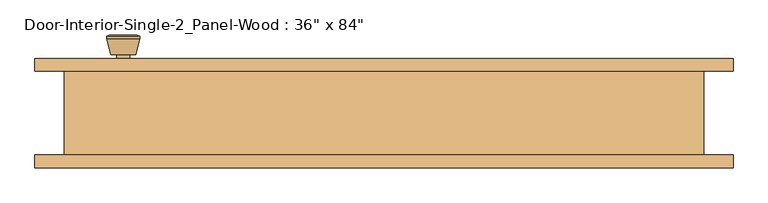
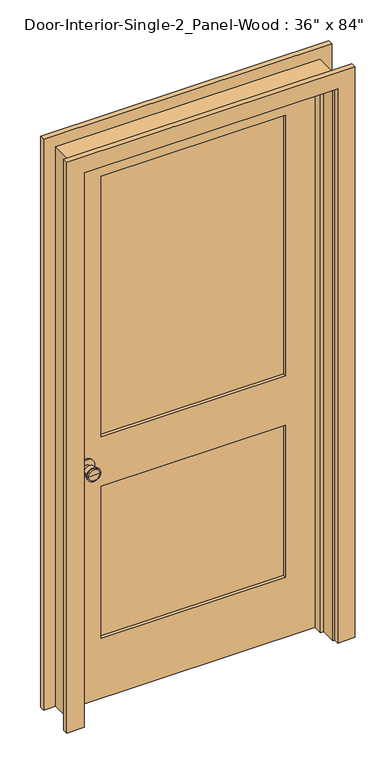
"""IFC4 building model written with IfcOpenShell, lengths in millimetres: door geometry."""

from ifc_helpers import new_model, si_unit, point, frame, frame_2d, origin, place, context, project, spatial, polyline, circle_curve, trimmed, segment, composite_curve, outline, extrude, faceted_brep, source, transform, mapped, element, save
from ifc_brep_helpers import plane_surface, cylinder_surface, revolved_surface, advanced_brep


def door_9f0e9c7d(model_context):
    return source(origin(), model_context, "Body", "SolidModel", [
        advanced_brep(
        [(-393.7, 19.4, 914.4), (-383.7, 19.4, 914.4), (-403.7, 19.4, 914.4), (-373.2241324, -29.6, 914.4), (-393.7, -29.6, 914.4), (-414.1758676, -29.6, 914.4), (-368.7, -27.7721319, 914.4), (-418.7, -27.7721319, 914.4), (-368.7, -24.3084537, 914.4), (-418.7, -24.3084537, 914.4), (-375.063764, 0.4, 914.4), (-412.336236, 0.4, 914.4), (-383.7, 0.4, 914.4), (-403.7, 0.4, 914.4)],
        [
            (0, 1),
            (1, 2, circle_curve(frame((-393.7, 19.4, 914.4), z_axis=(0.0, 1.0, 0.0), x_axis=(-1.0, 0.0, 0.0)), 10.0)),
            (2, 0),
            (2, 1, circle_curve(frame((-393.7, 19.4, 914.4), z_axis=(0.0, 1.0, 0.0), x_axis=(-1.0, 0.0, 0.0)), 10.0)),
            (3, 4),
            (4, 5),
            (5, 3, circle_curve(frame((-393.7, -29.6, 914.4), z_axis=(0.0, -1.0, 0.0), x_axis=(-1.0, 0.0, 0.0)), 20.4758676)),
            (3, 5, circle_curve(frame((-393.7, -29.6, 914.4), z_axis=(0.0, -1.0, 0.0), x_axis=(-1.0, 0.0, 0.0)), 20.4758676)),
            (6, 3),
            (5, 7),
            (7, 6, circle_curve(frame((-393.7, -27.7721319, 914.4), z_axis=(0.0, -1.0, 0.0), x_axis=(-1.0, 0.0, 0.0)), 25.0)),
            (6, 7, circle_curve(frame((-393.7, -27.7721319, 914.4), z_axis=(0.0, -1.0, 0.0), x_axis=(-1.0, 0.0, 0.0)), 25.0)),
            (8, 6),
            (7, 9),
            (9, 8, circle_curve(frame((-393.7, -24.3084537, 914.4), z_axis=(0.0, -1.0, 0.0), x_axis=(-1.0, 0.0, 0.0)), 25.0)),
            (8, 9, circle_curve(frame((-393.7, -24.3084537, 914.4), z_axis=(0.0, -1.0, 0.0), x_axis=(-1.0, 0.0, 0.0)), 25.0)),
            (10, 8),
            (9, 11),
            (11, 10, circle_curve(frame((-393.7, 0.4, 914.4), z_axis=(0.0, -1.0, 0.0), x_axis=(-1.0, 0.0, 0.0)), 18.636236)),
            (10, 11, circle_curve(frame((-393.7, 0.4, 914.4), z_axis=(0.0, -1.0, 0.0), x_axis=(-1.0, 0.0, 0.0)), 18.636236)),
            (12, 10),
            (11, 13),
            (13, 12, circle_curve(frame((-393.7, 0.4, 914.4), z_axis=(0.0, -1.0, 0.0), x_axis=(-1.0, 0.0, 0.0)), 10.0)),
            (12, 13, circle_curve(frame((-393.7, 0.4, 914.4), z_axis=(0.0, -1.0, 0.0), x_axis=(-1.0, 0.0, 0.0)), 10.0)),
            (1, 12),
            (13, 2),
        ],
        [
            plane_surface(frame((-393.7, 19.4, 914.4), z_axis=(0.0, 1.0, 0.0), x_axis=(-1.0, 0.0, 0.0))),
            plane_surface(frame((-393.7, -29.6, 914.4), z_axis=(0.0, -1.0, 0.0), x_axis=(-1.0, 0.0, 0.0))),
            revolved_surface(polyline([(-414.1758676, -29.6, 914.4), (-418.7, -27.7721319, 914.4)]), (-393.7, 19.4, 914.4), (0.0, 1.0, 0.0)),
            cylinder_surface(frame((-393.7, 19.4, 914.4), z_axis=(0.0, 1.0, 0.0), x_axis=(-1.0, 0.0, 0.0)), 25.0),
            revolved_surface(polyline([(-418.7, -24.3084537, 914.4), (-412.336236, 0.4, 914.4)]), (-393.7, 19.4, 914.4), (0.0, 1.0, 0.0)),
            plane_surface(frame((-393.7, 0.4, 914.4), z_axis=(0.0, 1.0, 0.0), x_axis=(-1.0, 0.0, 0.0))),
            cylinder_surface(frame((-393.7, 19.4, 914.4), z_axis=(0.0, 1.0, 0.0), x_axis=(-1.0, 0.0, 0.0)), 10.0),
        ],
        [
            (0, [[1, 2, 3]]),
            (0, [[-3, 4, -1]]),
            (1, [[5, 6, 7]]),
            (1, [[-6, -5, 8]]),
            (2, [[9, -7, 10, 11]]),
            (2, [[-10, -8, -9, 12]]),
            (3, [[13, -11, 14, 15]]),
            (3, [[-14, -12, -13, 16]]),
            (4, [[17, -15, 18, 19]]),
            (4, [[-18, -16, -17, 20]]),
            (5, [[21, -19, 22, 23]]),
            (5, [[-22, -20, -21, 24]]),
            (6, [[25, -23, 26, -2]]),
            (6, [[-26, -24, -25, -4]]),
        ],
    ),
        extrude(outline(composite_curve([segment(trimmed(circle_curve(frame_2d((914.4, -393.7)), 30.0), [point((914.4, -423.7))], [point((914.4, -363.7))], False, "CARTESIAN"), True, "CONTINUOUS"), segment(trimmed(circle_curve(frame_2d((914.4, -393.7)), 30.0), [point((914.4, -363.7))], [point((914.4, -423.7))], False, "CARTESIAN"), True, "CONTINUOUS")], self_intersect=False)), frame((0.0, 19.4, 0.0), z_axis=(0.0, 1.0, 0.0), x_axis=(0.0, 0.0, 1.0)), (0.0, 0.0, 1.0), 6.0),
        advanced_brep(
        [(-393.7, 66.325, 914.4), (-403.7, 66.325, 914.4), (-383.7, 66.325, 914.4), (-373.2241324, 115.325, 914.4), (-414.1758676, 115.325, 914.4), (-393.7, 115.325, 914.4), (-368.7, 113.4971319, 914.4), (-418.7, 113.4971319, 914.4), (-368.7, 110.0334537, 914.4), (-418.7, 110.0334537, 914.4), (-375.063764, 85.325, 914.4), (-412.336236, 85.325, 914.4), (-383.7, 85.325, 914.4), (-403.7, 85.325, 914.4)],
        [
            (0, 1),
            (1, 2, circle_curve(frame((-393.7, 66.325, 914.4), z_axis=(0.0, -1.0, 0.0), x_axis=(-1.0, 0.0, 0.0)), 10.0)),
            (2, 0),
            (2, 1, circle_curve(frame((-393.7, 66.325, 914.4), z_axis=(0.0, -1.0, 0.0), x_axis=(-1.0, 0.0, 0.0)), 10.0)),
            (3, 4, circle_curve(frame((-393.7, 115.325, 914.4), z_axis=(0.0, 1.0, 0.0), x_axis=(-1.0, 0.0, 0.0)), 20.4758676)),
            (4, 5),
            (5, 3),
            (4, 3, circle_curve(frame((-393.7, 115.325, 914.4), z_axis=(0.0, 1.0, 0.0), x_axis=(-1.0, 0.0, 0.0)), 20.4758676)),
            (6, 7, circle_curve(frame((-393.7, 113.4971319, 914.4), z_axis=(0.0, 1.0, 0.0), x_axis=(-1.0, 0.0, 0.0)), 25.0)),
            (7, 4),
            (3, 6),
            (7, 6, circle_curve(frame((-393.7, 113.4971319, 914.4), z_axis=(0.0, 1.0, 0.0), x_axis=(-1.0, 0.0, 0.0)), 25.0)),
            (8, 9, circle_curve(frame((-393.7, 110.0334537, 914.4), z_axis=(0.0, 1.0, 0.0), x_axis=(-1.0, 0.0, 0.0)), 25.0)),
            (9, 7),
            (6, 8),
            (9, 8, circle_curve(frame((-393.7, 110.0334537, 914.4), z_axis=(0.0, 1.0, 0.0), x_axis=(-1.0, 0.0, 0.0)), 25.0)),
            (10, 11, circle_curve(frame((-393.7, 85.325, 914.4), z_axis=(0.0, 1.0, 0.0), x_axis=(-1.0, 0.0, 0.0)), 18.636236)),
            (11, 9),
            (8, 10),
            (11, 10, circle_curve(frame((-393.7, 85.325, 914.4), z_axis=(0.0, 1.0, 0.0), x_axis=(-1.0, 0.0, 0.0)), 18.636236)),
            (12, 13, circle_curve(frame((-393.7, 85.325, 914.4), z_axis=(0.0, 1.0, 0.0), x_axis=(-1.0, 0.0, 0.0)), 10.0)),
            (13, 11),
            (10, 12),
            (13, 12, circle_curve(frame((-393.7, 85.325, 914.4), z_axis=(0.0, 1.0, 0.0), x_axis=(-1.0, 0.0, 0.0)), 10.0)),
            (1, 13),
            (12, 2),
        ],
        [
            plane_surface(frame((-393.7, 66.325, 914.4), z_axis=(0.0, -1.0, 0.0), x_axis=(-1.0, 0.0, 0.0))),
            plane_surface(frame((-393.7, 115.325, 914.4), z_axis=(0.0, 1.0, 0.0), x_axis=(-1.0, 0.0, 0.0))),
            revolved_surface(polyline([(-414.1758676, 115.325, 914.4), (-418.7, 113.4971319, 914.4)]), (-393.7, 66.325, 914.4), (0.0, -1.0, 0.0)),
            cylinder_surface(frame((-393.7, 66.325, 914.4), z_axis=(0.0, -1.0, 0.0), x_axis=(-1.0, 0.0, 0.0)), 25.0),
            revolved_surface(polyline([(-418.7, 110.0334537, 914.4), (-412.336236, 85.325, 914.4)]), (-393.7, 66.325, 914.4), (0.0, -1.0, 0.0)),
            plane_surface(frame((-393.7, 85.325, 914.4), z_axis=(0.0, -1.0, 0.0), x_axis=(-1.0, 0.0, 0.0))),
            cylinder_surface(frame((-393.7, 66.325, 914.4), z_axis=(0.0, -1.0, 0.0), x_axis=(-1.0, 0.0, 0.0)), 10.0),
        ],
        [
            (0, [[1, 2, 3]]),
            (0, [[-3, 4, -1]]),
            (1, [[5, 6, 7]]),
            (1, [[8, -7, -6]]),
            (2, [[9, 10, -5, 11]]),
            (2, [[12, -11, -8, -10]]),
            (3, [[13, 14, -9, 15]]),
            (3, [[16, -15, -12, -14]]),
            (4, [[17, 18, -13, 19]]),
            (4, [[20, -19, -16, -18]]),
            (5, [[21, 22, -17, 23]]),
            (5, [[24, -23, -20, -22]]),
            (6, [[-2, 25, -21, 26]]),
            (6, [[-4, -26, -24, -25]]),
        ],
    ),
        extrude(outline(composite_curve([segment(trimmed(circle_curve(frame_2d((914.4, -393.7)), 30.0), [point((914.4, -423.7))], [point((914.4, -363.7))], False, "CARTESIAN"), True, "CONTINUOUS"), segment(trimmed(circle_curve(frame_2d((914.4, -393.7)), 30.0), [point((914.4, -363.7))], [point((914.4, -423.7))], False, "CARTESIAN"), True, "CONTINUOUS")], self_intersect=False)), frame((0.0, 60.325, 0.0), z_axis=(0.0, 1.0, 0.0), x_axis=(0.0, 0.0, 1.0)), (0.0, 0.0, 1.0), 6.0),
        extrude(outline(polyline([(336.55, 37.0416667), (-336.55, 37.0416667), (-336.55, 48.6833333), (336.55, 48.6833333), (336.55, 37.0416667)])), frame((0.0, 0.0, 1009.65), z_axis=(0.0, 0.0, 1.0), x_axis=(1.0, 0.0, 0.0)), (0.0, 0.0, 1.0), 1004.8875),
        extrude(outline(polyline([(336.55, 37.0416667), (-336.55, 37.0416667), (-336.55, 48.6833333), (336.55, 48.6833333), (336.55, 37.0416667)])), frame((0.0, 0.0, 231.775), z_axis=(0.0, 0.0, 1.0), x_axis=(1.0, 0.0, 0.0)), (0.0, 0.0, 1.0), 587.375),
        extrude(outline(polyline([(2133.6, -457.2), (0.0, -457.2), (0.0, 457.2), (2133.6, 457.2), (2133.6, -457.2)]), holes=[polyline([(2014.5375, -336.55), (2014.5375, 336.55), (1009.65, 336.55), (1009.65, -336.55), (2014.5375, -336.55)]), polyline([(819.15, -336.55), (819.15, 336.55), (231.775, 336.55), (231.775, -336.55), (819.15, -336.55)])]), frame((0.0, 25.4, 0.0), z_axis=(0.0, 1.0, 0.0), x_axis=(0.0, 0.0, 1.0)), (0.0, 0.0, 1.0), 34.925),
        faceted_brep([(482.6, 60.325, 0.0), (482.6, -66.675, 0.0), (457.2, -66.675, 0.0), (457.2, -9.525, 0.0), (444.5, -9.525, 0.0), (444.5, 25.4, 0.0), (457.2, 25.4, 0.0), (457.2, 60.325, 0.0), (482.6, 60.325, 2159.0), (482.6, -66.675, 2159.0), (-482.6, -66.675, 2159.0), (-482.6, -66.675, 0.0), (-457.2, -66.675, 0.0), (-457.2, -66.675, 2133.6), (457.2, -66.675, 2133.6), (457.2, -9.525, 2133.6), (-457.2, -9.525, 2133.6), (-457.2, -9.525, 0.0), (-444.5, -9.525, 0.0), (-444.5, -9.525, 2120.9), (444.5, -9.525, 2120.9), (444.5, 25.4, 2120.9), (-444.5, 25.4, 2120.9), (-444.5, 25.4, 0.0), (-457.2, 25.4, 0.0), (-457.2, 25.4, 2133.6), (457.2, 25.4, 2133.6), (457.2, 60.325, 2133.6), (-457.2, 60.325, 2133.6), (-457.2, 60.325, 0.0), (-482.6, 60.325, 0.0), (-482.6, 60.325, 2159.0)], [[[0, 1, 2, 3, 4, 5, 6, 7]], [[1, 0, 8, 9]], [[2, 1, 9, 10, 11, 12, 13, 14]], [[3, 2, 14, 15]], [[4, 3, 15, 16, 17, 18, 19, 20]], [[5, 4, 20, 21]], [[6, 5, 21, 22, 23, 24, 25, 26]], [[7, 6, 26, 27]], [[0, 7, 27, 28, 29, 30, 31, 8]], [[9, 8, 31, 10]], [[15, 14, 13, 16]], [[21, 20, 19, 22]], [[27, 26, 25, 28]], [[30, 29, 24, 23, 18, 17, 12, 11]], [[10, 31, 30, 11]], [[16, 13, 12, 17]], [[22, 19, 18, 23]], [[28, 25, 24, 29]]]),
        extrude(outline(polyline([(0.0, 463.55), (0.0, 527.05), (2203.45, 527.05), (2203.45, -527.05), (0.0, -527.05), (0.0, -463.55), (2139.95, -463.55), (2139.95, 463.55), (0.0, 463.55)])), frame((0.0, -85.725, 0.0), z_axis=(0.0, 1.0, 0.0), x_axis=(0.0, 0.0, 1.0)), (0.0, 0.0, 1.0), 19.05),
        extrude(outline(polyline([(0.0, 463.55), (0.0, 527.05), (2203.45, 527.05), (2203.45, -527.05), (0.0, -527.05), (0.0, -463.55), (2139.95, -463.55), (2139.95, 463.55), (0.0, 463.55)])), frame((0.0, 60.325, 0.0), z_axis=(0.0, 1.0, 0.0), x_axis=(0.0, 0.0, 1.0)), (0.0, 0.0, 1.0), 19.05),
    ])


if __name__ == "__main__":
    model = new_model("IFC4")
    model_context = context("Model", 3, world=origin())
    ifc_project = project(units=[si_unit("LENGTHUNIT", "METRE", prefix="MILLI")], contexts=[model_context])
    site = spatial("IfcSite", under=ifc_project)
    building = spatial("IfcBuilding", under=site)
    placement = place(None, origin())
    door_shape = door_9f0e9c7d(model_context)
    element("IfcDoor", 1, ObjectType="Door-Interior-Single-2_Panel-Wood : 36\" x 84\"", at=placement, inside=building, context=model_context, shape_type="MappedRepresentation", body=[
        mapped(door_shape, transform((0.0, 0.0, 0.0), x_axis=(1.0, 0.0, 0.0), y_axis=(0.0, 1.0, 0.0), z_axis=(0.0, 0.0, 1.0))),
    ])
    save(model, "model.ifc")

# Revit data of these elements
# Type "Door-Interior-Single-2_Panel-Wood : 36\" x 84\""
#   Type Mark = "17"
#   Assembly Code = "C1020300"
#   Analytic Construction = "Wooden"
#   Top Rail = 0' - 4 11/16"
#   Thickness = 0' - 1 3/8"
#   Thermal Resistance (R) = 2.5876 (h·ft²·°F)/BTU
#   Swing Angle [instance default] = 90.00°
#   Stiles = 0' - 4 3/4"
#   Rough Width = 3' - 2"
#   Rough Height = 7' - 1"
#   Lock Rail = 0' - 7 1/2"
#   Height = 7' - 0"
#   Width = 3' - 0"
#   Heat Transfer Coefficient (U) = 0.3865 BTU/(h·ft²·°F)
#   Bottom Rail = 0' - 9 1/8"
#   Function = 0
#   Define Thermal Properties by = 1
#   Trim Material = Cherry
#   Panel Material = Cherry
#   Frame Material = Cherry
#   Door Handle Material = Aluminum
#   Visual Light Transmittance = 0
#   Solar Heat Gain Coefficient = 0
#   Wall Closure = (empty or 0)
#   Function = (empty or 0)
# Element 1 (IfcDoor, "Door-Interior-Single-2_Panel-Wood : 36\" x 84\"")
#   Materials on its faces: "Cherry", "Aluminum"
# Materials
#   "Cherry": class "Wood", colour RGB 157 77 38, transparency 0, Description = "Prunus Serotina", Cost = 0
#   "Aluminum": class "Metal", colour RGB 120 120 120, transparency 0, Description = "Aluminum 6061", Cost = 0
